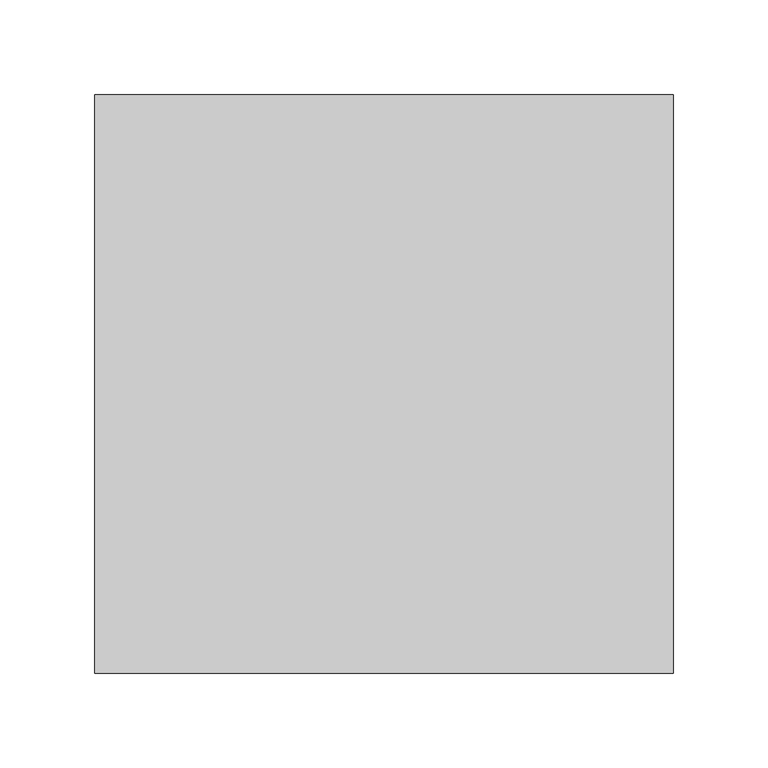
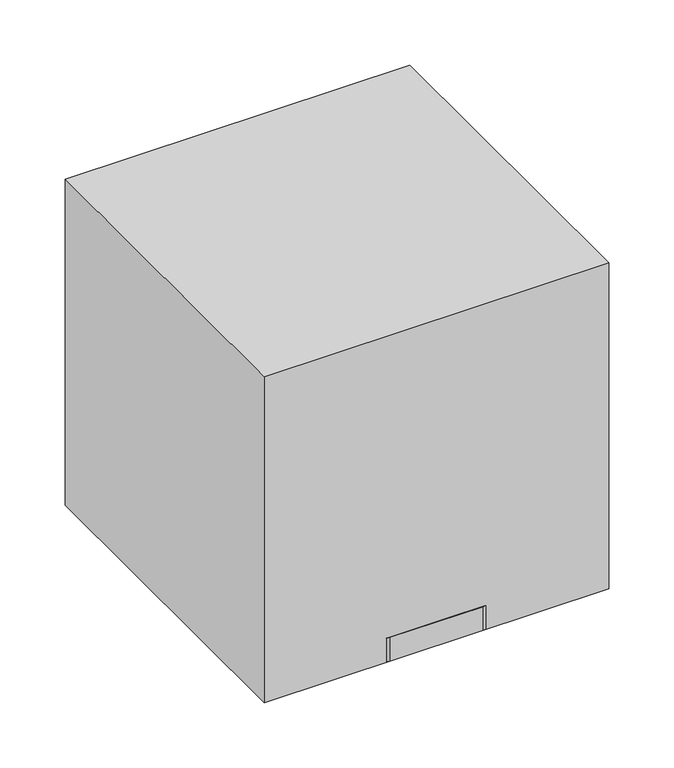
"""IFC4 building model written with IfcOpenShell, lengths in millimetres: proxy geometry, A5140 - Hook, Garment, Security : A5140 - Hook, Garment, Security."""

from ifc_helpers import new_model, si_unit, point, frame, frame_2d, origin, origin_with_axes, origin_2d, place, context, project, spatial, polyline, circle_curve, ellipse_curve, trimmed, segment, composite_curve, outline, extrude, source, transform, mapped, element, save
from ifc_brep_helpers import plane_surface, revolved_surface, advanced_brep


def specialty_equipment_5596d368(model_context):
    return source(origin(), model_context, "Body", "SolidModel", [
        extrude(outline(composite_curve([segment(trimmed(circle_curve(origin_2d(), 1.5875), [point((0.0, 1.5875))], [point((0.0, -1.5875001))], False, "CARTESIAN"), True, "CONTINUOUS"), segment(trimmed(circle_curve(origin_2d(), 1.5875), [point((0.0, -1.5875001))], [point((0.0, 1.5875))], False, "CARTESIAN"), True, "CONTINUOUS")], self_intersect=False)), frame((0.0, 55.6532473, 31.0200167), z_axis=(0.0, 0.4226182617407002, 0.9063077870366497), x_axis=(1.0, 0.0, 0.0)), (0.0, 0.0, 1.0), 25.4),
        advanced_brep(
        [(9.4955556, 53.975, 22.225), (-9.4955556, 53.975, 22.225), (0.0, 53.975, 31.7205556), (0.0, 53.975, 22.225)],
        [
            (0, 1, circle_curve(frame((0.0, 53.975, 22.225), z_axis=(0.0, 0.0, 1.0), x_axis=(-1.0, 0.0, 0.0)), 9.4955556)),
            (1, 2, circle_curve(frame((0.0, 53.975, 22.225), z_axis=(0.0, 1.0, 0.0), x_axis=(1.0, 0.0, 0.0)), 9.4955556)),
            (2, 0, circle_curve(frame((0.0, 53.975, 22.225), z_axis=(0.0, 1.0, 0.0), x_axis=(-1.0, 0.0, 0.0)), 9.4955556)),
            (1, 0, circle_curve(frame((0.0, 53.975, 22.225), z_axis=(0.0, 0.0, 1.0), x_axis=(-1.0, 0.0, 0.0)), 9.4955556)),
            (3, 1),
            (0, 3),
        ],
        [
            revolved_surface(trimmed(ellipse_curve(frame((0.0, 53.975, 22.225), z_axis=(0.0, -1.0, 0.0), x_axis=(1.0, 0.0, 0.0)), 9.4955556, 9.4955556), [point((0.0, 53.975, 31.7205556))], [point((-9.4955556, 53.975, 22.225))], True, "CARTESIAN"), (0.0, 53.975, 31.7205556), (0.0, 0.0, -1.0)),
            plane_surface(frame((0.0, 53.975, 22.225), z_axis=(0.0, 0.0, -1.0), x_axis=(-1.0, 0.0, 0.0))),
        ],
        [
            (0, [[1, 2, 3]]),
            (0, [[4, -3, -2]]),
            (1, [[5, -1, 6]]),
            (1, [[-6, -4, -5]]),
        ],
    ),
        extrude(outline(composite_curve([segment(polyline([(41.275, 0.0), (-41.275, 0.0)]), True, "CONTINUOUS"), segment(trimmed(circle_curve(frame_2d((-41.275, 12.7)), 12.7), [point((-41.275, 0.0))], [point((-53.975, 12.7))], False, "CARTESIAN"), True, "CONTINUOUS"), segment(polyline([(-53.975, 12.7), (-53.975, 95.25)]), True, "CONTINUOUS"), segment(trimmed(circle_curve(frame_2d((-41.275, 95.25)), 12.7), [point((-53.975, 95.25))], [point((-41.275, 107.95))], False, "CARTESIAN"), True, "CONTINUOUS"), segment(polyline([(-41.275, 107.95), (41.275, 107.95)]), True, "CONTINUOUS"), segment(trimmed(circle_curve(frame_2d((41.275, 95.25)), 12.7), [point((41.275, 107.95))], [point((53.975, 95.25))], False, "CARTESIAN"), True, "CONTINUOUS"), segment(polyline([(53.975, 95.25), (53.975, 12.7)]), True, "CONTINUOUS"), segment(trimmed(circle_curve(frame_2d((41.275, 12.7)), 12.7), [point((53.975, 12.7))], [point((41.275, 0.0))], False, "CARTESIAN"), True, "CONTINUOUS")], self_intersect=False)), origin_with_axes(), (0.0, 0.0, 1.0), 22.225),
        extrude(outline(polyline([(152.4, 304.8), (152.4, 0.0), (-152.4, 0.0), (-152.4, 304.8), (152.4, 304.8)])), origin_with_axes(), (0.0, 0.0, 1.0), 304.8),
    ])


if __name__ == "__main__":
    model = new_model("IFC4")
    model_context = context("Model", 3, world=origin())
    ifc_project = project(units=[si_unit("LENGTHUNIT", "METRE", prefix="MILLI")], contexts=[model_context])
    site = spatial("IfcSite", under=ifc_project)
    building = spatial("IfcBuilding", under=site)
    placement = place(None, origin())
    specialty_equipment_shape = specialty_equipment_5596d368(model_context)
    element("IfcBuildingElementProxy", 1, Name="A5140 - Hook, Garment, Security : A5140 - Hook, Garment, Security", ObjectType="A5140 - Hook, Garment, Security : A5140 - Hook, Garment, Security", at=placement, inside=building, context=model_context, shape_type="MappedRepresentation", body=[
        mapped(specialty_equipment_shape, transform((0.0, 0.0, 0.0), x_axis=(1.0, 0.0, 0.0), y_axis=(0.0, 1.0, 0.0), z_axis=(0.0, 0.0, 1.0))),
    ])
    save(model, "model.ifc")

# Revit data of these elements
# Project information
#   Room Abbreviation = "BRNP2/TLTP3"
#   Room Description 2-1 = "Bedroom, Behavioral Health (Double Occupancy) (BRNP2)"
#   Room Description 2-2 = "Toilet/Shower, Behavioral Health (TLTP3)"
#   Sheets - Total = "6"
#   Project Issue Date = "Issue Date"
#   Project Status = "Project Status"
#   Client Name = "Owner"
#   Project Address = "Enter address here"
#   Project Name = "Project Name"
#   Project Number = "Project Number"
#   Publication Date = "1-Feb-16"
# Type "A5140 - Hook, Garment, Security : A5140 - Hook, Garment, Security"
#   Watts2 = "0"
#   Watts1 = "0"
#   Unit_Issue = "EA"
#   UTIL_6_Misc = "-"
#   UTIL_5_NonMedGas = "-"
#   UTIL_4_MiscGas = "-"
#   UTIL_3_MedGas = "-"
#   UTIL_2_Elec = "-"
#   UTIL_1_WaterDrain = "-"
#   Nomenclature = "Hook, Garment, Security"
#   NSN = ""
#   Location [instance default] = ""
#   JSN = "A5140"
#   Fund_Source_VA = "-"
#   Fund_Source_Navy = "-"
#   Fund_Source_Army = "-"
#   Fund_Source_AF = "-"
#   ELEC_Volts2 = "0"
#   ELEC_Volts1 = "0"
#   ELEC_Phase2 = "0"
#   ELEC_Phase1 = "0"
#   ELEC_HertzSwitch = "0"
#   ELEC_HertzDependent = "0"
#   ELEC_Hertz = "0"
#   ELEC_Amps2 = "0"
#   ELEC_Amps1 = "0"
#   DetailDescription = "Clothes hook used in patient rooms of psychiatric, drug abuse or alcohol rehab facilities."
#   CAT_VA = "A"
#   CAT_Navy = "A"
#   CAT_IHS = "-"
#   CAT_Army = "A"
#   CAT_AF = "A"
#   BTUperhour = "0"
#   Weight_IP = 2
#   Default Elevation = 4' - 0"
#   DIM_Width_IP = 1' - 0"
#   DIM_Height_IP = 1' - 0"
#   DIM_Depth_IP = 1' - 0"
# Element 1 (IfcBuildingElementProxy, "A5140 - Hook, Garment, Security : A5140 - Hook, Garment, Security")
#   Materials on its faces: "EquipSpace"
# Materials
#   "EquipSpace": class "Unassigned", colour RGB 221 217 195, transparency 0.5
